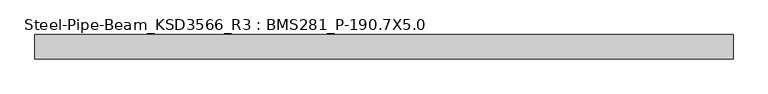
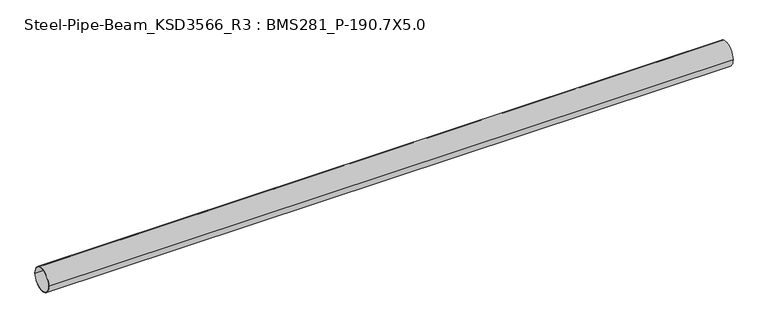
"""IFC4 building model written with IfcOpenShell, lengths in millimetres: member geometry, Steel-Pipe-Beam_KSD3566_R3 : BMS281_P-190.7X5.0."""

from ifc_helpers import new_model, si_unit, point, frame, origin, origin_2d, place, context, project, spatial, circle_curve, trimmed, segment, composite_curve, outline, extrude, source, transform, mapped, element, save


def steel_pipe_beam_ksd3566_r3_bms281_p_190_7x5_0_cc3e612d(model_context):
    return source(origin(), model_context, "Body", "SweptSolid", [
        extrude(outline(composite_curve([segment(trimmed(circle_curve(origin_2d(), 95.35), [point((-95.35, 0.0))], [point((95.35, 0.0))], False, "CARTESIAN"), True, "CONTINUOUS"), segment(trimmed(circle_curve(origin_2d(), 95.35), [point((95.35, 0.0))], [point((-95.35, 0.0))], False, "CARTESIAN"), True, "CONTINUOUS")], self_intersect=False), holes=[composite_curve([segment(trimmed(circle_curve(origin_2d(), 90.35), [point((90.35, 0.0))], [point((-90.35, 0.0))], True, "CARTESIAN"), True, "CONTINUOUS"), segment(trimmed(circle_curve(origin_2d(), 90.35), [point((-90.35, 0.0))], [point((90.35, 0.0))], True, "CARTESIAN"), True, "CONTINUOUS")], self_intersect=False)]), frame((-2725.3244663, 0.0, 0.0), z_axis=(1.0, 0.0, 0.0), x_axis=(0.0, 1.0, 0.0)), (0.0, 0.0, 1.0), 5477.7690397),
    ])


if __name__ == "__main__":
    model = new_model("IFC4")
    model_context = context("Model", 3, world=origin())
    ifc_project = project(units=[si_unit("LENGTHUNIT", "METRE", prefix="MILLI")], contexts=[model_context])
    site = spatial("IfcSite", under=ifc_project)
    building = spatial("IfcBuilding", under=site)
    placement = place(None, origin())
    steel_pipe_beam_ksd3566_r3_bms281_p_190_7x5_0_shape = steel_pipe_beam_ksd3566_r3_bms281_p_190_7x5_0_cc3e612d(model_context)
    element("IfcMember", 1, ObjectType="Steel-Pipe-Beam_KSD3566_R3 : BMS281_P-190.7X5.0", at=placement, inside=building, context=model_context, shape_type="MappedRepresentation", body=[
        mapped(steel_pipe_beam_ksd3566_r3_bms281_p_190_7x5_0_shape, transform((0.0, 0.0, 0.0), x_axis=(1.0, 0.0, 0.0), y_axis=(0.0, 1.0, 0.0), z_axis=(0.0, 0.0, 1.0))),
    ])
    save(model, "model.ifc")

# Revit data of these elements
# Type "Steel-Pipe-Beam_KSD3566_R3 : BMS281_P-190.7X5.0"
#   Keynote = "P-190.7X5.0"
#   SteelWeight = "Light"
#   t = 0.0050 m
#   Surface Area = 0.599102 m²/m
#   Section Area = 29.1697 cm²
#   Mass per Unit Length = 22.8982 kg/m
#   Length [instance default] = 1.5000 m
#   D = 0.1907 m
#   hec_material4 [instance default] = none
#   hec_material3 [instance default] = none
#   hec_material2 [instance default] = none
#   hec_material1 [instance default] = none
#   Structural Material [instance default] = Steel, 45-345
#   Assembly Code = ""
# Element 1 (IfcMember, "Steel-Pipe-Beam_KSD3566_R3 : BMS281_P-190.7X5.0")
#   Structural Material = none
# Materials
#   "Steel, 45-345": class "Metal", colour RGB 189 187 185, transparency 0, Description = "Steel 345 MPa", Cost = 0
